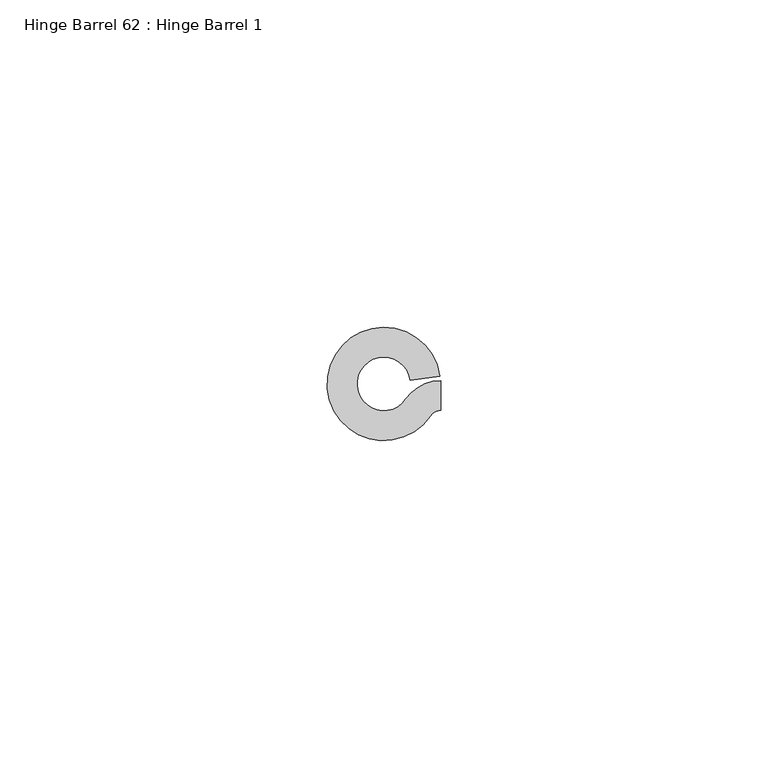
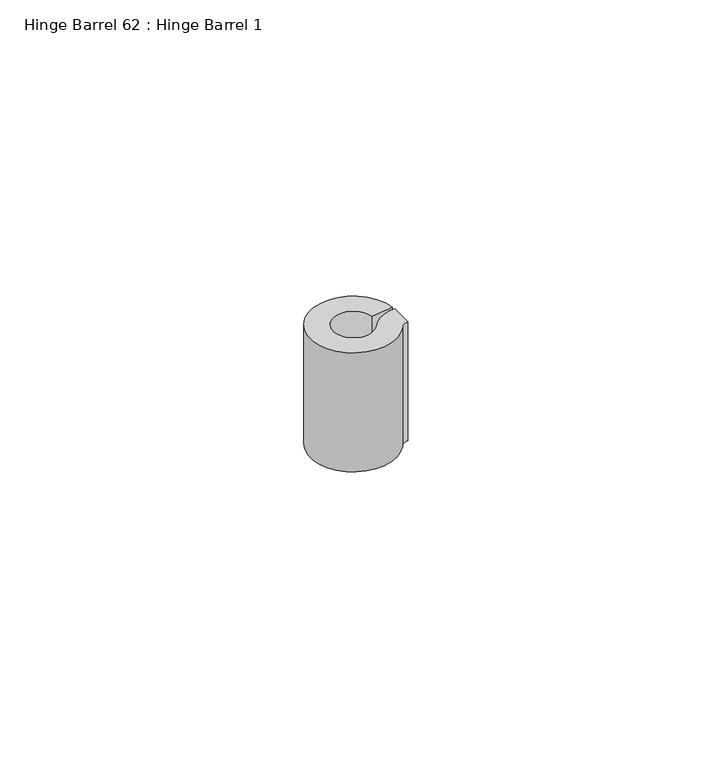
"""IFC4 building model written with IfcOpenShell, lengths in millimetres: proxy geometry, Hinge Barrel 62 : Hinge Barrel 1."""

from ifc_helpers import new_model, si_unit, point, frame, frame_2d, origin, place, context, project, spatial, polyline, circle_curve, trimmed, segment, composite_curve, outline, extrude, source, transform, mapped, element, save


def hinge_barrel_62_hinge_barrel_1_ef8cf91d(model_context):
    return source(origin(), model_context, "Body", "SweptSolid", [
        extrude(outline(composite_curve([segment(trimmed(circle_curve(frame_2d((587327.8245257, -536316.2443067)), 6.4044851), [point((587322.5194669, -536312.6563017))], [point((587327.8245257, -536309.8398216))], False, "CARTESIAN"), True, "CONTINUOUS"), segment(polyline([(587327.8245257, -536309.8398216), (587327.8245257, -536314.4038841)]), True, "CONTINUOUS"), segment(trimmed(circle_curve(frame_2d((587327.8245257, -536316.2443067)), 1.8404226), [point((587327.8245257, -536314.4038841))], [point((587326.3000393, -536315.2132409))], True, "CARTESIAN"), True, "CONTINUOUS"), segment(trimmed(circle_curve(frame_2d((587319.1320739, -536310.3652841)), 8.6534625), [point((587326.3000393, -536315.2132409))], [point((587327.7022899, -536309.1678654))], False, "CARTESIAN"), True, "CONTINUOUS"), segment(polyline([(587327.7022899, -536309.1678654), (587323.1821338, -536309.7994153)]), True, "CONTINUOUS"), segment(trimmed(circle_curve(frame_2d((587319.1320739, -536310.3652841)), 4.0894), [point((587323.1821338, -536309.7994153))], [point((587322.5194669, -536312.6563017))], True, "CARTESIAN"), True, "CONTINUOUS")], self_intersect=False)), frame((0.0, 0.0, 1962.15), z_axis=(0.0, 0.0, 1.0), x_axis=(1.0, 0.0, 0.0)), (0.0, 0.0, 1.0), 25.4),
    ])


if __name__ == "__main__":
    model = new_model("IFC4")
    model_context = context("Model", 3, world=origin())
    ifc_project = project(units=[si_unit("LENGTHUNIT", "METRE", prefix="MILLI")], contexts=[model_context])
    site = spatial("IfcSite", under=ifc_project)
    building = spatial("IfcBuilding", under=site)
    placement = place(None, origin())
    hinge_barrel_62_hinge_barrel_1_shape = hinge_barrel_62_hinge_barrel_1_ef8cf91d(model_context)
    element("IfcBuildingElementProxy", 1, Name="Hinge Barrel 62 : Hinge Barrel 1", ObjectType="Hinge Barrel 62 : Hinge Barrel 1", at=placement, inside=building, context=model_context, shape_type="MappedRepresentation", body=[
        mapped(hinge_barrel_62_hinge_barrel_1_shape, transform((0.0, 0.0, 0.0), x_axis=(1.0, 0.0, 0.0), y_axis=(0.0, 1.0, 0.0), z_axis=(0.0, 0.0, 1.0))),
    ])
    save(model, "model.ifc")

# Revit data of these elements
# Element 1 (IfcBuildingElementProxy, "Hinge Barrel 62 : Hinge Barrel 1")
#   Materials on its faces: "6\"X6\" WELD-ON STL BUTT HINGE"
# Materials
#   "6\"X6\" WELD-ON STL BUTT HINGE": class "Metal", colour RGB 189 187 185, transparency 0, Description = "Carbon steel", Cost = 0
